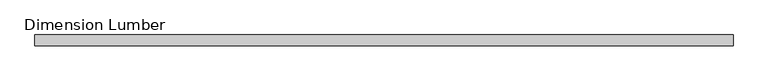
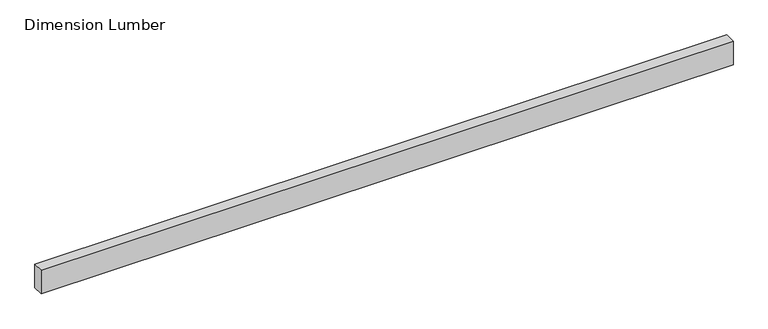
"""IFC4 building model written with IfcOpenShell, lengths in millimetres: beam geometry, Dimension Lumber : Roof Lumbers."""

from ifc_helpers import new_model, si_unit, frame, origin, place, context, project, spatial, polyline, outline, extrude, source, transform, mapped, element, save


def dimension_lumber_70fa0837(model_context):
    return source(origin(), model_context, "Body", "SweptSolid", [
        extrude(outline(polyline([(1250.4988621, 19.05), (1250.4988621, -19.05), (-1214.6940206, -19.05), (-1214.6940206, 19.05), (1250.4988621, 19.05)])), frame((0.0, 0.0, -44.45), z_axis=(0.0, 0.0, 1.0), x_axis=(1.0, 0.0, 0.0)), (0.0, 0.0, 1.0), 88.9),
    ])


if __name__ == "__main__":
    model = new_model("IFC4")
    model_context = context("Model", 3, world=origin())
    ifc_project = project(units=[si_unit("LENGTHUNIT", "METRE", prefix="MILLI")], contexts=[model_context])
    site = spatial("IfcSite", under=ifc_project)
    building = spatial("IfcBuilding", under=site)
    placement = place(None, origin())
    dimension_lumber_shape = dimension_lumber_70fa0837(model_context)
    element("IfcBeam", 1, ObjectType="Dimension Lumber : Roof Lumbers", at=placement, inside=building, context=model_context, shape_type="MappedRepresentation", body=[
        mapped(dimension_lumber_shape, transform((0.0, 0.0, 0.0), x_axis=(1.0, 0.0, 0.0), y_axis=(0.0, 1.0, 0.0), z_axis=(0.0, 0.0, 1.0))),
    ])
    save(model, "model.ifc")

# Revit data of these elements
# Type "Dimension Lumber : Roof Lumbers"
#   Assembly Code = "B10"
#   A = 0.0364583 SF
#   Length [instance default] = 5' - 0"
#   b = 0' - 1 1/2"
#   d = 0' - 3 1/2"
#   Structural Material [instance default] = Softwood, Lumber
# Element 1 (IfcBeam, "Dimension Lumber : Roof Lumbers")
#   Materials on its faces: "Softwood, Lumber"
# Materials
#   "Softwood, Lumber": class "Wood", colour RGB 223 192 134, transparency 0, Description = "Pinus Echinata", Cost = 0
